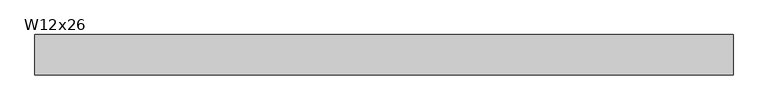
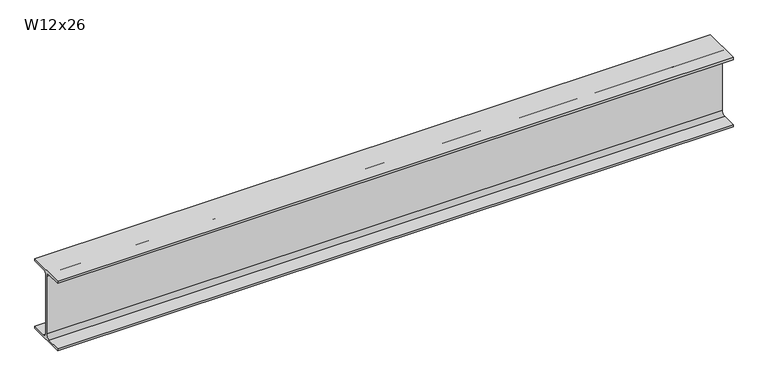
"""IFC4 building model written with IfcOpenShell, lengths in millimetres: beam geometry, RME W-Wide Flange : W12x26."""

from ifc_helpers import new_model, si_unit, point, frame, frame_2d, origin, place, context, project, spatial, polyline, circle_curve, trimmed, segment, composite_curve, outline, extrude, source, transform, mapped, element, save


def w12x26_ff4ea4fa(model_context):
    return source(origin(), model_context, "Body", "SweptSolid", [
        extrude(outline(composite_curve([segment(polyline([(82.423, -145.288), (82.423, -154.94), (-82.423, -154.94), (-82.423, -145.288), (-20.2565, -145.288)]), True, "CONTINUOUS"), segment(trimmed(circle_curve(frame_2d((-20.2565, -127.9525)), 17.3355), [point((-20.2565, -145.288))], [point((-2.921, -127.9525))], True, "CARTESIAN"), True, "CONTINUOUS"), segment(polyline([(-2.921, -127.9525), (-2.921, 127.9525)]), True, "CONTINUOUS"), segment(trimmed(circle_curve(frame_2d((-20.2565, 127.9525)), 17.3355), [point((-2.921, 127.9525))], [point((-20.2565, 145.288))], True, "CARTESIAN"), True, "CONTINUOUS"), segment(polyline([(-20.2565, 145.288), (-82.423, 145.288), (-82.423, 154.94), (82.423, 154.94), (82.423, 145.288), (20.2565, 145.288)]), True, "CONTINUOUS"), segment(trimmed(circle_curve(frame_2d((20.2565, 127.9525)), 17.3355), [point((20.2565, 145.288))], [point((2.921, 127.9525))], True, "CARTESIAN"), True, "CONTINUOUS"), segment(polyline([(2.921, 127.9525), (2.921, -127.9525)]), True, "CONTINUOUS"), segment(trimmed(circle_curve(frame_2d((20.2565, -127.9525)), 17.3355), [point((2.921, -127.9525))], [point((20.2565, -145.288))], True, "CARTESIAN"), True, "CONTINUOUS"), segment(polyline([(20.2565, -145.288), (82.423, -145.288)]), True, "CONTINUOUS")], self_intersect=False)), frame((-1421.1119873, 0.0, 0.0), z_axis=(1.0, 0.0, 0.0), x_axis=(0.0, 1.0, 0.0)), (0.0, 0.0, 1.0), 2845.1737825),
    ])


if __name__ == "__main__":
    model = new_model("IFC4")
    model_context = context("Model", 3, world=origin())
    ifc_project = project(units=[si_unit("LENGTHUNIT", "METRE", prefix="MILLI")], contexts=[model_context])
    site = spatial("IfcSite", under=ifc_project)
    building = spatial("IfcBuilding", under=site)
    placement = place(None, origin())
    w12x26_shape = w12x26_ff4ea4fa(model_context)
    element("IfcBeam", 1, ObjectType="RME W-Wide Flange : W12x26", at=placement, inside=building, context=model_context, shape_type="MappedRepresentation", body=[
        mapped(w12x26_shape, transform((0.0, 0.0, 0.0), x_axis=(1.0, 0.0, 0.0), y_axis=(0.0, 1.0, 0.0), z_axis=(0.0, 0.0, 1.0))),
    ])
    save(model, "model.ifc")

# Revit data of these elements
# Type "RME W-Wide Flange : W12x26"
#   WELD P [instance default] = ""
#   WELD LE [instance default] = ""
#   WELD D [instance default] = ""
#   TOP SECTION SIZE [instance default] = ""
#   TOP SECTION LENGTH [instance default] = ""
#   REMARKS [instance default] = ""
#   REINF TYPE [instance default] = ""
#   Nominal Size = "W24"
#   End Bearing Capacity [instance default] = ""
#   BOT SECTION SIZE [instance default] = ""
#   BOT SECTION LENGTH [instance default] = ""
#   Assembly Code = "B10"
#   W = 26
#   Start Extension Calculation [instance default] = 10' - 0"
#   Start Extension [instance default] = -0' - 0 1/2"
#   End Extension Calculation [instance default] = 10' - 0"
#   End Extension [instance default] = -0' - 0 1/2"
#   Length [instance default] = 5' - 0"
#   bf = 0' - 6.49"
#   d = 1' - 0.2"
#   k = 0' - 1 1/16"
#   k2 = 0' - 0.6825"
#   tf = 0' - 0.38"
#   tw = 0' - 0.23"
#   A = 0.053125 SF
#   Structural Material [instance default] = Metal - Steel - ASTM A992
# Element 1 (IfcBeam, "RME W-Wide Flange : W12x26")
#   Length = 9' - 4.13085"
#   Materials on its faces: "Metal - Steel - ASTM A992"
# Materials
#   "Metal - Steel - ASTM A992": class "Metal", colour RGB 255 128 0, transparency 0
